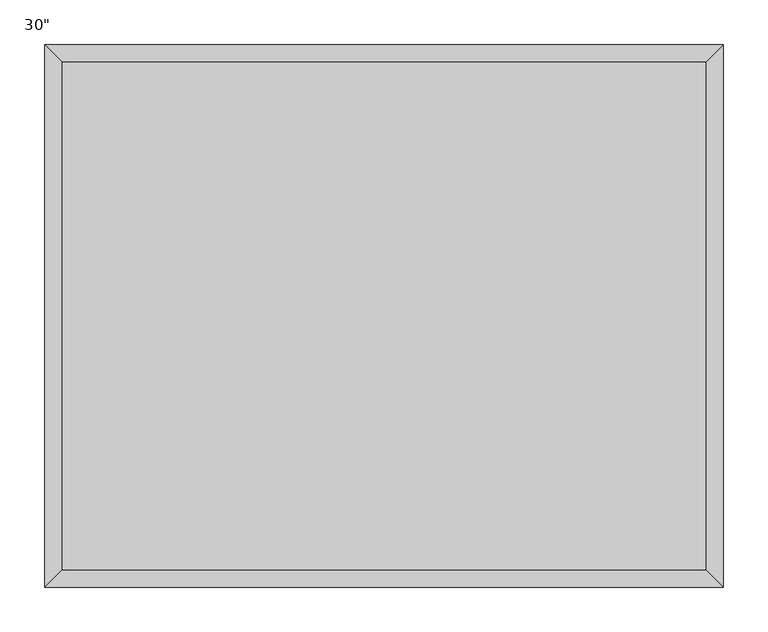
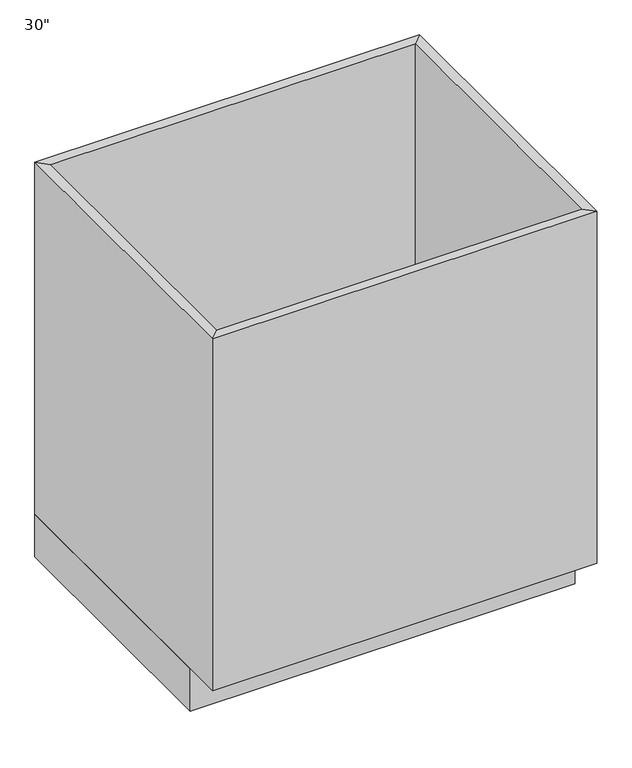
"""IFC4 building model written with IfcOpenShell, lengths in millimetres: furniture geometry."""

import ifcopenshell
import ifcopenshell.guid

model = None  # the IFC model being written
_history = None  # IfcOwnerHistory: only IFC2X3 demands one
_inside = {}  # id of a spatial element -> (the spatial element, [elements in it])
_under = {}  # id of a project, library or spatial element -> (it, [spatial elements below it])
_declared = {}  # id of a project -> (the project, [libraries it declares])
_typed = {}  # id of a type object -> (the type object, [elements of that type])
_made_of = {}  # id of a material, layer set ... -> (it, [elements and type objects made of it])


def new_model(schema):
    """Start an empty IFC model of exactly this schema.

    Asked for "IFC4X3", IfcOpenShell would pick the latest addendum, in which some entities
    have other attributes; the version numbers below select the first issue.
    IFC2X3 requires an IfcOwnerHistory on every rooted entity: one is made here for all.
    """
    global model, _history
    if schema == "IFC4X3":
        model = ifcopenshell.file(schema_version=(4, 3, 0, 0))
    else:
        model = ifcopenshell.file(schema=schema)
    _inside.clear()
    _under.clear()
    _declared.clear()
    _typed.clear()
    _made_of.clear()
    _history = None
    if model.schema == "IFC2X3":
        org = make("IfcOrganization", Name="unknown")
        user = make(
            "IfcPersonAndOrganization",
            ThePerson=make("IfcPerson", FamilyName="unknown"),
            TheOrganization=org,
        )
        app = make(
            "IfcApplication",
            ApplicationDeveloper=org,
            Version="unknown",
            ApplicationFullName="unknown",
            ApplicationIdentifier="unknown",
        )
        _history = make(
            "IfcOwnerHistory",
            OwningUser=user,
            OwningApplication=app,
            ChangeAction="ADDED",
            CreationDate=0,
        )
    return model


def make(cls, **values):
    """One entity of the class cls with the attributes given. An attribute that is None is left unset."""
    return model.create_entity(
        cls, **{name: value for name, value in values.items() if value is not None}
    )


def rooted(cls, **values):
    """An entity with a GlobalId (a new one), such as an element, a storey or a relation."""
    return make(cls, GlobalId=ifcopenshell.guid.new(), OwnerHistory=_history, **values)


def si_unit(unit_type, name, prefix=None):
    """IfcSIUnit, for example si_unit("LENGTHUNIT", "METRE", prefix="MILLI")."""
    return make("IfcSIUnit", UnitType=unit_type, Prefix=prefix, Name=name)


def assignment(units):
    """IfcUnitAssignment: the units of a project."""
    return None if units is None else make("IfcUnitAssignment", Units=units)


def point(xyz):
    """IfcCartesianPoint."""
    return None if xyz is None else make("IfcCartesianPoint", Coordinates=xyz)


def direction(xyz):
    """IfcDirection."""
    return None if xyz is None else make("IfcDirection", DirectionRatios=xyz)


def frame(location, z_axis=None, x_axis=None):
    """IfcAxis2Placement3D, a coordinate frame: its origin and axes. An axis left out is left unset."""
    return make(
        "IfcAxis2Placement3D",
        Location=point(location),
        Axis=direction(z_axis),
        RefDirection=direction(x_axis),
    )


def origin():
    """The frame at (0, 0, 0) with its axes left unset."""
    return frame((0.0, 0.0, 0.0))


def origin_with_axes():
    """The frame at (0, 0, 0) with the z axis (0, 0, 1) and the x axis (1, 0, 0) written out."""
    return frame((0.0, 0.0, 0.0), z_axis=(0.0, 0.0, 1.0), x_axis=(1.0, 0.0, 0.0))


def place(relative_to, where):
    """IfcLocalPlacement: puts the frame where relative to a parent placement (None: the world)."""
    return make(
        "IfcLocalPlacement", PlacementRelTo=relative_to, RelativePlacement=where
    )


def context(
    kind, dimensions, precision=None, world=None, true_north=None, identifier=None
):
    """IfcGeometricRepresentationContext, for example the 3D "Model" context."""
    return make(
        "IfcGeometricRepresentationContext",
        ContextIdentifier=identifier,
        ContextType=kind,
        CoordinateSpaceDimension=dimensions,
        Precision=precision,
        WorldCoordinateSystem=world,
        TrueNorth=true_north,
    )


def project(units=None, contexts=None):
    """IfcProject with its units and contexts."""
    return rooted(
        "IfcProject",
        Name="project",
        RepresentationContexts=contexts,
        UnitsInContext=assignment(units),
    )


def spatial(cls, under=None, at=None, **own):
    """A site, building, storey or space (cls), placed at a placement, below another one or the project."""
    s = rooted(cls, ObjectPlacement=at, **own)
    if under is not None:
        _under.setdefault(under.id(), (under, []))[1].append(s)
    return s


def polyline(points):
    """IfcPolyline through the points."""
    return make("IfcPolyline", Points=[point(p) for p in points])


def outline(outer, holes=None, kind="AREA"):
    """IfcArbitraryClosedProfileDef: a profile drawn as a closed curve; with holes, ...WithVoids."""
    if holes is None:
        return make("IfcArbitraryClosedProfileDef", ProfileType=kind, OuterCurve=outer)
    return make(
        "IfcArbitraryProfileDefWithVoids",
        ProfileType=kind,
        OuterCurve=outer,
        InnerCurves=holes,
    )


def extrude(swept, where, along, depth):
    """IfcExtrudedAreaSolid: the profile swept, set in the frame where, extruded along a direction by depth."""
    return make(
        "IfcExtrudedAreaSolid",
        SweptArea=swept,
        Position=where,
        ExtrudedDirection=direction(along),
        Depth=depth,
    )


def faces_of(points, faces, orient=None, outer=None):
    """IfcFace entities. A face is a list of loops; a loop is a list of indices into points, from 0.

    orient and outer hold one flag for each loop. By default every Orientation is true, the
    first loop of a face is its IfcFaceOuterBound and the others are IfcFaceBound.
    """
    made = []
    for i, loops in enumerate(faces):
        bounds = []
        for j, loop in enumerate(loops):
            is_outer = j == 0 if outer is None else outer[i][j]
            bounds.append(
                make(
                    "IfcFaceOuterBound" if is_outer else "IfcFaceBound",
                    Bound=make("IfcPolyLoop", Polygon=[points[k] for k in loop]),
                    Orientation=True if orient is None else orient[i][j],
                )
            )
        made.append(make("IfcFace", Bounds=bounds))
    return made


def faceted_brep(points, faces, orient=None, outer=None, voids=None):
    """IfcFacetedBrep: a solid bounded by flat faces; with voids (closed shells), ...WithVoids."""
    shared = [point(p) for p in points]
    hull = make("IfcClosedShell", CfsFaces=faces_of(shared, faces, orient, outer))
    if voids is None:
        return make("IfcFacetedBrep", Outer=hull)
    return make(
        "IfcFacetedBrepWithVoids",
        Outer=hull,
        Voids=[
            make(cls, CfsFaces=faces_of(shared, fs, o, b)) for cls, fs, o, b in voids
        ],
    )


def shape(context_of_items, identifier, shape_type, items):
    """IfcShapeRepresentation: the items that make up one representation, for example the "Body"."""
    return make(
        "IfcShapeRepresentation",
        ContextOfItems=context_of_items,
        RepresentationIdentifier=identifier,
        RepresentationType=shape_type,
        Items=items,
    )


def source(mapping_origin, context_of_items, identifier, shape_type, items):
    """IfcRepresentationMap: a shape defined once, which mapped items show again and again."""
    return make(
        "IfcRepresentationMap",
        MappingOrigin=mapping_origin,
        MappedRepresentation=shape(context_of_items, identifier, shape_type, items),
    )


def transform(
    local_origin,
    x_axis=None,
    y_axis=None,
    z_axis=None,
    scale=None,
    scale2=None,
    scale3=None,
    uniform=True,
):
    """IfcCartesianTransformationOperator3D, or its non-uniform kind. x_axis, y_axis, z_axis: its Axis1, 2, 3."""
    if uniform:
        return make(
            "IfcCartesianTransformationOperator3D",
            Axis1=direction(x_axis),
            Axis2=direction(y_axis),
            LocalOrigin=point(local_origin),
            Scale=scale,
            Axis3=direction(z_axis),
        )
    return make(
        "IfcCartesianTransformationOperator3DnonUniform",
        Axis1=direction(x_axis),
        Axis2=direction(y_axis),
        LocalOrigin=point(local_origin),
        Scale=scale,
        Axis3=direction(z_axis),
        Scale2=scale2,
        Scale3=scale3,
    )


def mapped(mapping_source, mapping_target):
    """IfcMappedItem: shows the shape of a source again, moved by a transform."""
    return make(
        "IfcMappedItem", MappingSource=mapping_source, MappingTarget=mapping_target
    )


def made_of(thing, what):
    """Note that an element or type object is made of a material, layer set ...; save() writes the relation."""
    if what is not None:
        _made_of.setdefault(what.id(), (what, []))[1].append(thing)
    return thing


def element(
    cls,
    number,
    at=None,
    inside=None,
    cuts=None,
    type_object=None,
    material=None,
    context=None,
    identifier="Body",
    shape_type=None,
    held_by="IfcProductDefinitionShape",
    body=None,
    shapes=None,
    **own,
):
    """One element of the class cls, such as IfcWall. Its Tag is "e" and its number.

    at: its placement. inside: the storey or other place that contains it. cuts: it is an
    opening in that element (IfcRelVoidsElement). A single representation is given by context,
    identifier, shape_type and body (its items); several are given by shapes. held_by: the class
    of the entity that holds the representations. save() writes the other relations.
    """
    e = rooted(cls, Tag="e%d" % number, ObjectPlacement=at, **own)
    if body is not None:
        shapes = [shape(context, identifier, shape_type, body)]
    if shapes is not None:
        e.Representation = make(held_by, Representations=shapes)
    if inside is not None:
        _inside.setdefault(inside.id(), (inside, []))[1].append(e)
    if cuts is not None:
        rooted(
            "IfcRelVoidsElement", RelatingBuildingElement=cuts, RelatedOpeningElement=e
        )
    if type_object is not None:
        _typed.setdefault(type_object.id(), (type_object, []))[1].append(e)
    return made_of(e, material)


def aggregate(whole, parts):
    """IfcRelAggregates: a whole, such as a stair, and the parts it consists of."""
    return rooted("IfcRelAggregates", RelatingObject=whole, RelatedObjects=parts)


def save(model, path):
    """Write the relations noted so far, then the file.

    IfcRelAggregates (storeys below a building ...), IfcRelContainedInSpatialStructure (elements
    in a storey), IfcRelDefinesByType, IfcRelAssociatesMaterial and IfcRelDeclares: one each for
    every whole, place, type object, material and project.
    """
    for whole, parts in _under.values():
        aggregate(whole, parts)
    for where, things in _inside.values():
        rooted(
            "IfcRelContainedInSpatialStructure",
            RelatedElements=things,
            RelatingStructure=where,
        )
    for kind, things in _typed.values():
        rooted("IfcRelDefinesByType", RelatedObjects=things, RelatingType=kind)
    for what, things in _made_of.values():
        rooted("IfcRelAssociatesMaterial", RelatedObjects=things, RelatingMaterial=what)
    for by, libraries in _declared.values():
        rooted("IfcRelDeclares", RelatingContext=by, RelatedDefinitions=libraries)
    model.write(path)


def furniture_6ba5c079(model_context):
    return source(origin(), model_context, "Body", "SolidModel", [
        extrude(outline(polyline([(380.6877049, -19.05), (380.6877049, -590.55), (-343.2122951, -590.55), (-343.2122951, -19.05), (380.6877049, -19.05)])), frame((0.0, 0.0, 88.9), z_axis=(0.0, 0.0, 1.0), x_axis=(1.0, 0.0, 0.0)), (0.0, 0.0, 1.0), 19.05),
        faceted_brep([(380.6877049, -590.55, 825.5), (380.6877049, -590.55, 88.9), (-343.2122951, -590.55, 88.9), (-343.2122951, -590.55, 825.5), (399.7377049, -609.6, 825.5), (-362.2622951, -609.6, 825.5), (399.7377049, -609.6, 88.9), (-362.2622951, -609.6, 88.9), (-343.2122951, -19.05, 88.9), (-343.2122951, -19.05, 825.5), (-362.2622951, 0.0, 825.5), (-362.2622951, 0.0, 88.9), (380.6877049, -19.05, 88.9), (380.6877049, -19.05, 825.5), (399.7377049, 0.0, 825.5), (399.7377049, 0.0, 88.9)], [[[0, 1, 2, 3]], [[4, 0, 3, 5]], [[6, 4, 5, 7]], [[1, 6, 7, 2]], [[3, 2, 8, 9]], [[5, 3, 9, 10]], [[7, 5, 10, 11]], [[2, 7, 11, 8]], [[9, 8, 12, 13]], [[10, 9, 13, 14]], [[11, 10, 14, 15]], [[8, 11, 15, 12]], [[13, 12, 1, 0]], [[14, 13, 0, 4]], [[15, 14, 4, 6]], [[12, 15, 6, 1]]]),
        extrude(outline(polyline([(399.7377049, 0.0), (399.7377049, -533.4), (-362.2622951, -533.4), (-362.2622951, 0.0), (399.7377049, 0.0)])), origin_with_axes(), (0.0, 0.0, 1.0), 88.9),
    ])


if __name__ == "__main__":
    model = new_model("IFC4")
    model_context = context("Model", 3, world=origin())
    ifc_project = project(units=[si_unit("LENGTHUNIT", "METRE", prefix="MILLI")], contexts=[model_context])
    site = spatial("IfcSite", under=ifc_project)
    building = spatial("IfcBuilding", under=site)
    placement = place(None, origin())
    furniture_shape = furniture_6ba5c079(model_context)
    element("IfcFurniture", 1, ObjectType="Base Cabinet-Double Door & 1 Drawer : 30\"", at=placement, inside=building, context=model_context, shape_type="MappedRepresentation", body=[
        mapped(furniture_shape, transform((0.0, 0.0, 0.0), x_axis=(1.0, 0.0, 0.0), y_axis=(0.0, 1.0, 0.0), z_axis=(0.0, 0.0, 1.0))),
    ])
    save(model, "model.ifc")

# Revit data of these elements
# Type "Base Cabinet-Double Door & 1 Drawer : 30\""
#   Finish = "Cabinetry"
#   Finish = "Cabinet"
#   Depth = 2' - 0"
#   Height = 2' - 8 1/2"
#   Toe Depth = 0' - 3"
#   Toe Height = 0' - 3 1/2"
#   Width = 2' - 6"
#   Cabinet Material = none
# Element 1 (IfcFurniture, "Base Cabinet-Double Door & 1 Drawer : 30\"")
#   Materials on its faces: "MAX HEIGHT OF  COUNTERTOP 34\""
# Materials
#   "MAX HEIGHT OF  COUNTERTOP 34\"": class "Generic", colour RGB 181 181 181, transparency 0, Cost = 0
